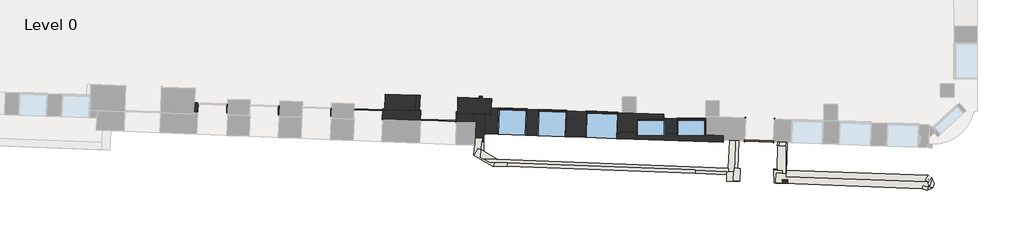
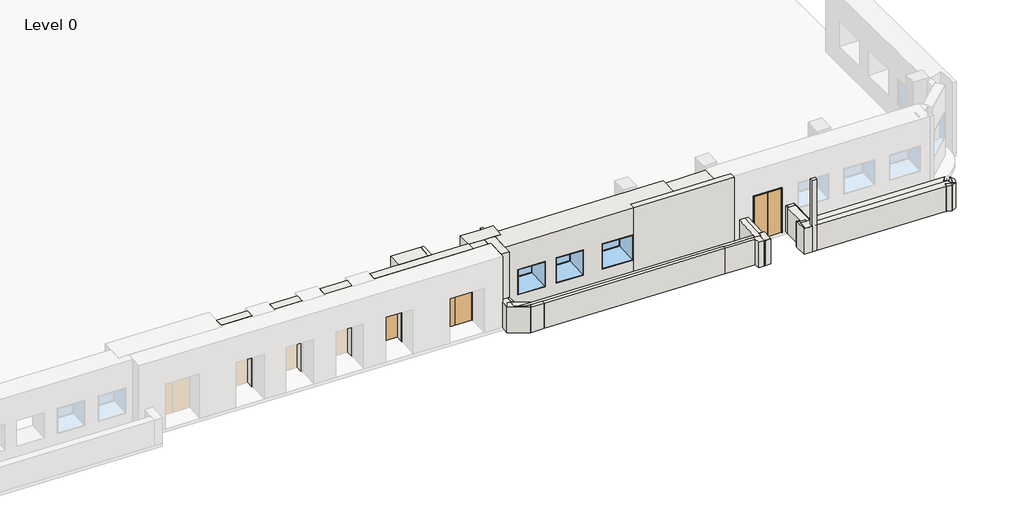
# One storey, part 2 of 9: 37 walls, 5 windows, 3 doors.
"""IFC4 building model written with IfcOpenShell, lengths in millimetres."""

import ifcopenshell
import ifcopenshell.guid

model = None  # the IFC model being written
_history = None  # IfcOwnerHistory: only IFC2X3 demands one
_inside = {}  # id of a spatial element -> (the spatial element, [elements in it])
_under = {}  # id of a project, library or spatial element -> (it, [spatial elements below it])
_declared = {}  # id of a project -> (the project, [libraries it declares])
_typed = {}  # id of a type object -> (the type object, [elements of that type])
_made_of = {}  # id of a material, layer set ... -> (it, [elements and type objects made of it])


def new_model(schema):
    """Start an empty IFC model of exactly this schema.

    Asked for "IFC4X3", IfcOpenShell would pick the latest addendum, in which some entities
    have other attributes; the version numbers below select the first issue.
    IFC2X3 requires an IfcOwnerHistory on every rooted entity: one is made here for all.
    """
    global model, _history
    if schema == "IFC4X3":
        model = ifcopenshell.file(schema_version=(4, 3, 0, 0))
    else:
        model = ifcopenshell.file(schema=schema)
    _inside.clear()
    _under.clear()
    _declared.clear()
    _typed.clear()
    _made_of.clear()
    _history = None
    if model.schema == "IFC2X3":
        org = make("IfcOrganization", Name="unknown")
        user = make(
            "IfcPersonAndOrganization",
            ThePerson=make("IfcPerson", FamilyName="unknown"),
            TheOrganization=org,
        )
        app = make(
            "IfcApplication",
            ApplicationDeveloper=org,
            Version="unknown",
            ApplicationFullName="unknown",
            ApplicationIdentifier="unknown",
        )
        _history = make(
            "IfcOwnerHistory",
            OwningUser=user,
            OwningApplication=app,
            ChangeAction="ADDED",
            CreationDate=0,
        )
    return model


def make(cls, **values):
    """One entity of the class cls with the attributes given. An attribute that is None is left unset."""
    return model.create_entity(
        cls, **{name: value for name, value in values.items() if value is not None}
    )


def rooted(cls, **values):
    """An entity with a GlobalId (a new one), such as an element, a storey or a relation."""
    return make(cls, GlobalId=ifcopenshell.guid.new(), OwnerHistory=_history, **values)


def si_unit(unit_type, name, prefix=None):
    """IfcSIUnit, for example si_unit("LENGTHUNIT", "METRE", prefix="MILLI")."""
    return make("IfcSIUnit", UnitType=unit_type, Prefix=prefix, Name=name)


def assignment(units):
    """IfcUnitAssignment: the units of a project."""
    return None if units is None else make("IfcUnitAssignment", Units=units)


def point(xyz):
    """IfcCartesianPoint."""
    return None if xyz is None else make("IfcCartesianPoint", Coordinates=xyz)


def direction(xyz):
    """IfcDirection."""
    return None if xyz is None else make("IfcDirection", DirectionRatios=xyz)


def frame(location, z_axis=None, x_axis=None):
    """IfcAxis2Placement3D, a coordinate frame: its origin and axes. An axis left out is left unset."""
    return make(
        "IfcAxis2Placement3D",
        Location=point(location),
        Axis=direction(z_axis),
        RefDirection=direction(x_axis),
    )


def origin():
    """The frame at (0, 0, 0) with its axes left unset."""
    return frame((0.0, 0.0, 0.0))


def origin_with_axes():
    """The frame at (0, 0, 0) with the z axis (0, 0, 1) and the x axis (1, 0, 0) written out."""
    return frame((0.0, 0.0, 0.0), z_axis=(0.0, 0.0, 1.0), x_axis=(1.0, 0.0, 0.0))


def place(relative_to, where):
    """IfcLocalPlacement: puts the frame where relative to a parent placement (None: the world)."""
    return make(
        "IfcLocalPlacement", PlacementRelTo=relative_to, RelativePlacement=where
    )


def context(
    kind, dimensions, precision=None, world=None, true_north=None, identifier=None
):
    """IfcGeometricRepresentationContext, for example the 3D "Model" context."""
    return make(
        "IfcGeometricRepresentationContext",
        ContextIdentifier=identifier,
        ContextType=kind,
        CoordinateSpaceDimension=dimensions,
        Precision=precision,
        WorldCoordinateSystem=world,
        TrueNorth=true_north,
    )


def project(units=None, contexts=None):
    """IfcProject with its units and contexts."""
    return rooted(
        "IfcProject",
        Name="project",
        RepresentationContexts=contexts,
        UnitsInContext=assignment(units),
    )


def spatial(cls, under=None, at=None, **own):
    """A site, building, storey or space (cls), placed at a placement, below another one or the project."""
    s = rooted(cls, ObjectPlacement=at, **own)
    if under is not None:
        _under.setdefault(under.id(), (under, []))[1].append(s)
    return s


def polyline(points):
    """IfcPolyline through the points."""
    return make("IfcPolyline", Points=[point(p) for p in points])


def outline(outer, holes=None, kind="AREA"):
    """IfcArbitraryClosedProfileDef: a profile drawn as a closed curve; with holes, ...WithVoids."""
    if holes is None:
        return make("IfcArbitraryClosedProfileDef", ProfileType=kind, OuterCurve=outer)
    return make(
        "IfcArbitraryProfileDefWithVoids",
        ProfileType=kind,
        OuterCurve=outer,
        InnerCurves=holes,
    )


def extrude(swept, where, along, depth):
    """IfcExtrudedAreaSolid: the profile swept, set in the frame where, extruded along a direction by depth."""
    return make(
        "IfcExtrudedAreaSolid",
        SweptArea=swept,
        Position=where,
        ExtrudedDirection=direction(along),
        Depth=depth,
    )


def faces_of(points, faces, orient=None, outer=None):
    """IfcFace entities. A face is a list of loops; a loop is a list of indices into points, from 0.

    orient and outer hold one flag for each loop. By default every Orientation is true, the
    first loop of a face is its IfcFaceOuterBound and the others are IfcFaceBound.
    """
    made = []
    for i, loops in enumerate(faces):
        bounds = []
        for j, loop in enumerate(loops):
            is_outer = j == 0 if outer is None else outer[i][j]
            bounds.append(
                make(
                    "IfcFaceOuterBound" if is_outer else "IfcFaceBound",
                    Bound=make("IfcPolyLoop", Polygon=[points[k] for k in loop]),
                    Orientation=True if orient is None else orient[i][j],
                )
            )
        made.append(make("IfcFace", Bounds=bounds))
    return made


def faceted_brep(points, faces, orient=None, outer=None, voids=None):
    """IfcFacetedBrep: a solid bounded by flat faces; with voids (closed shells), ...WithVoids."""
    shared = [point(p) for p in points]
    hull = make("IfcClosedShell", CfsFaces=faces_of(shared, faces, orient, outer))
    if voids is None:
        return make("IfcFacetedBrep", Outer=hull)
    return make(
        "IfcFacetedBrepWithVoids",
        Outer=hull,
        Voids=[
            make(cls, CfsFaces=faces_of(shared, fs, o, b)) for cls, fs, o, b in voids
        ],
    )


def shape(context_of_items, identifier, shape_type, items):
    """IfcShapeRepresentation: the items that make up one representation, for example the "Body"."""
    return make(
        "IfcShapeRepresentation",
        ContextOfItems=context_of_items,
        RepresentationIdentifier=identifier,
        RepresentationType=shape_type,
        Items=items,
    )


def source(mapping_origin, context_of_items, identifier, shape_type, items):
    """IfcRepresentationMap: a shape defined once, which mapped items show again and again."""
    return make(
        "IfcRepresentationMap",
        MappingOrigin=mapping_origin,
        MappedRepresentation=shape(context_of_items, identifier, shape_type, items),
    )


def transform(
    local_origin,
    x_axis=None,
    y_axis=None,
    z_axis=None,
    scale=None,
    scale2=None,
    scale3=None,
    uniform=True,
):
    """IfcCartesianTransformationOperator3D, or its non-uniform kind. x_axis, y_axis, z_axis: its Axis1, 2, 3."""
    if uniform:
        return make(
            "IfcCartesianTransformationOperator3D",
            Axis1=direction(x_axis),
            Axis2=direction(y_axis),
            LocalOrigin=point(local_origin),
            Scale=scale,
            Axis3=direction(z_axis),
        )
    return make(
        "IfcCartesianTransformationOperator3DnonUniform",
        Axis1=direction(x_axis),
        Axis2=direction(y_axis),
        LocalOrigin=point(local_origin),
        Scale=scale,
        Axis3=direction(z_axis),
        Scale2=scale2,
        Scale3=scale3,
    )


def mapped(mapping_source, mapping_target):
    """IfcMappedItem: shows the shape of a source again, moved by a transform."""
    return make(
        "IfcMappedItem", MappingSource=mapping_source, MappingTarget=mapping_target
    )


def made_of(thing, what):
    """Note that an element or type object is made of a material, layer set ...; save() writes the relation."""
    if what is not None:
        _made_of.setdefault(what.id(), (what, []))[1].append(thing)
    return thing


def element(
    cls,
    number,
    at=None,
    inside=None,
    cuts=None,
    type_object=None,
    material=None,
    context=None,
    identifier="Body",
    shape_type=None,
    held_by="IfcProductDefinitionShape",
    body=None,
    shapes=None,
    **own,
):
    """One element of the class cls, such as IfcWall. Its Tag is "e" and its number.

    at: its placement. inside: the storey or other place that contains it. cuts: it is an
    opening in that element (IfcRelVoidsElement). A single representation is given by context,
    identifier, shape_type and body (its items); several are given by shapes. held_by: the class
    of the entity that holds the representations. save() writes the other relations.
    """
    e = rooted(cls, Tag="e%d" % number, ObjectPlacement=at, **own)
    if body is not None:
        shapes = [shape(context, identifier, shape_type, body)]
    if shapes is not None:
        e.Representation = make(held_by, Representations=shapes)
    if inside is not None:
        _inside.setdefault(inside.id(), (inside, []))[1].append(e)
    if cuts is not None:
        rooted(
            "IfcRelVoidsElement", RelatingBuildingElement=cuts, RelatedOpeningElement=e
        )
    if type_object is not None:
        _typed.setdefault(type_object.id(), (type_object, []))[1].append(e)
    return made_of(e, material)


def aggregate(whole, parts):
    """IfcRelAggregates: a whole, such as a stair, and the parts it consists of."""
    return rooted("IfcRelAggregates", RelatingObject=whole, RelatedObjects=parts)


def save(model, path):
    """Write the relations noted so far, then the file.

    IfcRelAggregates (storeys below a building ...), IfcRelContainedInSpatialStructure (elements
    in a storey), IfcRelDefinesByType, IfcRelAssociatesMaterial and IfcRelDeclares: one each for
    every whole, place, type object, material and project.
    """
    for whole, parts in _under.values():
        aggregate(whole, parts)
    for where, things in _inside.values():
        rooted(
            "IfcRelContainedInSpatialStructure",
            RelatedElements=things,
            RelatingStructure=where,
        )
    for kind, things in _typed.values():
        rooted("IfcRelDefinesByType", RelatedObjects=things, RelatingType=kind)
    for what, things in _made_of.values():
        rooted("IfcRelAssociatesMaterial", RelatedObjects=things, RelatingMaterial=what)
    for by, libraries in _declared.values():
        rooted("IfcRelDeclares", RelatingContext=by, RelatedDefinitions=libraries)
    model.write(path)


def door_1200x2100mm_edb93628(model_context):
    return source(origin(), model_context, "Body", "SweptSolid", [
        extrude(outline(polyline([(2125.0, -625.0), (0.0, -625.0), (0.0, -600.0), (2100.0, -600.0), (2100.0, 600.0), (0.0, 600.0), (0.0, 625.0), (2125.0, 625.0), (2125.0, -625.0)])), frame((0.0, 195.0, 0.0), z_axis=(0.0, 1.0, 0.0), x_axis=(0.0, 0.0, 1.0)), (0.0, 0.0, 1.0), 30.0),
        extrude(outline(polyline([(2125.0, 625.0), (2125.0, -625.0), (0.0, -625.0), (0.0, -600.0), (2100.0, -600.0), (2100.0, 600.0), (0.0, 600.0), (0.0, 625.0), (2125.0, 625.0)])), frame((0.0, -225.0, 0.0), z_axis=(0.0, 1.0, 0.0), x_axis=(0.0, 0.0, 1.0)), (0.0, 0.0, 1.0), 30.0),
        extrude(outline(polyline([(600.0, 145.0), (-600.0, 145.0), (-600.0, 195.0), (600.0, 195.0), (600.0, 145.0)])), origin_with_axes(), (0.0, 0.0, 1.0), 2100.0),
    ])


def door_1200x2100mm_3dafc3e4(model_context):
    return source(origin(), model_context, "Body", "SweptSolid", [
        extrude(outline(polyline([(0.0, 485.0), (600.0, 485.0), (600.0, 435.0), (0.0, 435.0), (0.0, 485.0)])), origin_with_axes(), (0.0, 0.0, 1.0), 2100.0),
        extrude(outline(polyline([(-600.0, 485.0), (0.0, 485.0), (0.0, 435.0), (-600.0, 435.0), (-600.0, 485.0)])), origin_with_axes(), (0.0, 0.0, 1.0), 2100.0),
        extrude(outline(polyline([(2100.0, -600.0), (2100.0, 600.0), (0.0, 600.0), (0.0, 625.0), (2125.0, 625.0), (2125.0, -625.0), (0.0, -625.0), (0.0, -600.0), (2100.0, -600.0)])), frame((0.0, -510.0, 0.0), z_axis=(0.0, 1.0, 0.0), x_axis=(0.0, 0.0, 1.0)), (0.0, 0.0, 1.0), 25.0),
        extrude(outline(polyline([(2100.0, -600.0), (2100.0, 600.0), (0.0, 600.0), (0.0, 625.0), (2125.0, 625.0), (2125.0, -625.0), (0.0, -625.0), (0.0, -600.0), (2100.0, -600.0)])), frame((0.0, 485.0, 0.0), z_axis=(0.0, 1.0, 0.0), x_axis=(0.0, 0.0, 1.0)), (0.0, 0.0, 1.0), 25.0),
    ])


def door_1500x2100mm_1360b9d6(model_context):
    return source(origin(), model_context, "Body", "SweptSolid", [
        extrude(outline(polyline([(0.0, 195.0), (750.0, 195.0), (750.0, 145.0), (0.0, 145.0), (0.0, 195.0)])), origin_with_axes(), (0.0, 0.0, 1.0), 2100.0),
        extrude(outline(polyline([(-750.0, 195.0), (0.0, 195.0), (0.0, 145.0), (-750.0, 145.0), (-750.0, 195.0)])), origin_with_axes(), (0.0, 0.0, 1.0), 2100.0),
        extrude(outline(polyline([(2100.0, -750.0), (2100.0, 750.0), (0.0, 750.0), (0.0, 775.0), (2125.0, 775.0), (2125.0, -775.0), (0.0, -775.0), (0.0, -750.0), (2100.0, -750.0)])), frame((0.0, -220.0, 0.0), z_axis=(0.0, 1.0, 0.0), x_axis=(0.0, 0.0, 1.0)), (0.0, 0.0, 1.0), 25.0),
        extrude(outline(polyline([(2100.0, -750.0), (2100.0, 750.0), (0.0, 750.0), (0.0, 775.0), (2125.0, 775.0), (2125.0, -775.0), (0.0, -775.0), (0.0, -750.0), (2100.0, -750.0)])), frame((0.0, 195.0, 0.0), z_axis=(0.0, 1.0, 0.0), x_axis=(0.0, 0.0, 1.0)), (0.0, 0.0, 1.0), 25.0),
    ])


def window_instance_600x1200_86a208f5(model_context):
    return source(origin(), model_context, "Body", "SweptSolid", [
        extrude(outline(polyline([(-713.1, 567.9), (636.9, 567.9), (636.9, 542.5), (-713.1, 542.5), (-713.1, 567.9)])), frame((0.0, 0.0, 900.0), z_axis=(0.0, 0.0, 1.0), x_axis=(1.0, 0.0, 0.0)), (0.0, 0.0, 1.0), 19.05),
        extrude(outline(polyline([(573.4, 493.925), (-649.6, 493.925), (-649.6, 506.625), (573.4, 506.625), (573.4, 493.925)])), frame((0.0, 0.0, 963.5), z_axis=(0.0, 0.0, 1.0), x_axis=(1.0, 0.0, 0.0)), (0.0, 0.0, 1.0), 1073.0),
        extrude(outline(polyline([(2080.95, -694.05), (919.05, -694.05), (919.05, 617.85), (2080.95, 617.85), (2080.95, -694.05)]), holes=[polyline([(2036.5, -649.6), (2036.5, 573.4), (963.5, 573.4), (963.5, -649.6), (2036.5, -649.6)])]), frame((0.0, 478.05, 0.0), z_axis=(0.0, 1.0, 0.0), x_axis=(0.0, 0.0, 1.0)), (0.0, 0.0, 1.0), 44.45),
        extrude(outline(polyline([(2100.0, -713.1), (900.0, -713.1), (900.0, 636.9), (2100.0, 636.9), (2100.0, -713.1)]), holes=[polyline([(2068.25, -681.35), (2068.25, 605.15), (931.75, 605.15), (931.75, -681.35), (2068.25, -681.35)])]), frame((0.0, -542.5, 0.0), z_axis=(0.0, 1.0, 0.0), x_axis=(0.0, 0.0, 1.0)), (0.0, 0.0, 1.0), 1020.55),
        extrude(outline(polyline([(2100.0, 636.9), (2100.0, -713.1), (900.0, -713.1), (900.0, 636.9), (2100.0, 636.9)]), holes=[polyline([(2080.95, 617.85), (919.05, 617.85), (919.05, -694.05), (2080.95, -694.05), (2080.95, 617.85)])]), frame((0.0, 478.05, 0.0), z_axis=(0.0, 1.0, 0.0), x_axis=(0.0, 0.0, 1.0)), (0.0, 0.0, 1.0), 64.45),
    ])


def window_instance_600x1200_c70fa3c9(model_context):
    return source(origin(), model_context, "Body", "SweptSolid", [
        extrude(outline(polyline([(-638.1, 382.9), (561.9, 382.9), (561.9, 357.5), (-638.1, 357.5), (-638.1, 382.9)])), frame((0.0, 0.0, 900.0), z_axis=(0.0, 0.0, 1.0), x_axis=(1.0, 0.0, 0.0)), (0.0, 0.0, 1.0), 19.05),
        extrude(outline(polyline([(498.4, 308.925), (-574.6, 308.925), (-574.6, 321.625), (498.4, 321.625), (498.4, 308.925)])), frame((0.0, 0.0, 963.5), z_axis=(0.0, 0.0, 1.0), x_axis=(1.0, 0.0, 0.0)), (0.0, 0.0, 1.0), 1073.0),
        extrude(outline(polyline([(2080.95, -619.05), (919.05, -619.05), (919.05, 542.85), (2080.95, 542.85), (2080.95, -619.05)]), holes=[polyline([(2036.5, -574.6), (2036.5, 498.4), (963.5, 498.4), (963.5, -574.6), (2036.5, -574.6)])]), frame((0.0, 293.05, 0.0), z_axis=(0.0, 1.0, 0.0), x_axis=(0.0, 0.0, 1.0)), (0.0, 0.0, 1.0), 44.45),
        extrude(outline(polyline([(2100.0, -638.1), (900.0, -638.1), (900.0, 561.9), (2100.0, 561.9), (2100.0, -638.1)]), holes=[polyline([(2068.25, -606.35), (2068.25, 530.15), (931.75, 530.15), (931.75, -606.35), (2068.25, -606.35)])]), frame((0.0, -357.5, 0.0), z_axis=(0.0, 1.0, 0.0), x_axis=(0.0, 0.0, 1.0)), (0.0, 0.0, 1.0), 650.55),
        extrude(outline(polyline([(2100.0, 561.9), (2100.0, -638.1), (900.0, -638.1), (900.0, 561.9), (2100.0, 561.9)]), holes=[polyline([(2080.95, 542.85), (919.05, 542.85), (919.05, -619.05), (2080.95, -619.05), (2080.95, 542.85)])]), frame((0.0, 293.05, 0.0), z_axis=(0.0, 1.0, 0.0), x_axis=(0.0, 0.0, 1.0)), (0.0, 0.0, 1.0), 64.45),
    ])


def window_instance_600x1200_b5ab94bb(model_context):
    return source(origin(), model_context, "Body", "SweptSolid", [
        extrude(outline(polyline([(-638.1, 567.9), (561.9, 567.9), (561.9, 542.5), (-638.1, 542.5), (-638.1, 567.9)])), frame((0.0, 0.0, 900.0), z_axis=(0.0, 0.0, 1.0), x_axis=(1.0, 0.0, 0.0)), (0.0, 0.0, 1.0), 19.05),
        extrude(outline(polyline([(498.4, 493.925), (-574.6, 493.925), (-574.6, 506.625), (498.4, 506.625), (498.4, 493.925)])), frame((0.0, 0.0, 963.5), z_axis=(0.0, 0.0, 1.0), x_axis=(1.0, 0.0, 0.0)), (0.0, 0.0, 1.0), 1073.0),
        extrude(outline(polyline([(2080.95, -619.05), (919.05, -619.05), (919.05, 542.85), (2080.95, 542.85), (2080.95, -619.05)]), holes=[polyline([(2036.5, -574.6), (2036.5, 498.4), (963.5, 498.4), (963.5, -574.6), (2036.5, -574.6)])]), frame((0.0, 478.05, 0.0), z_axis=(0.0, 1.0, 0.0), x_axis=(0.0, 0.0, 1.0)), (0.0, 0.0, 1.0), 44.45),
        extrude(outline(polyline([(2100.0, -638.1), (900.0, -638.1), (900.0, 561.9), (2100.0, 561.9), (2100.0, -638.1)]), holes=[polyline([(2068.25, -606.35), (2068.25, 530.15), (931.75, 530.15), (931.75, -606.35), (2068.25, -606.35)])]), frame((0.0, -542.5, 0.0), z_axis=(0.0, 1.0, 0.0), x_axis=(0.0, 0.0, 1.0)), (0.0, 0.0, 1.0), 1020.55),
        extrude(outline(polyline([(2100.0, 561.9), (2100.0, -638.1), (900.0, -638.1), (900.0, 561.9), (2100.0, 561.9)]), holes=[polyline([(2080.95, 542.85), (919.05, 542.85), (919.05, -619.05), (2080.95, -619.05), (2080.95, 542.85)])]), frame((0.0, 478.05, 0.0), z_axis=(0.0, 1.0, 0.0), x_axis=(0.0, 0.0, 1.0)), (0.0, 0.0, 1.0), 64.45),
    ])


model = new_model("IFC4")

# Units and contexts
model_context = context("Model", 3, world=origin())
ifc_project = project(units=[si_unit("LENGTHUNIT", "METRE", prefix="MILLI")], contexts=[model_context])

# Site, building, storey
site = spatial("IfcSite", under=ifc_project)
building = spatial("IfcBuilding", under=site)
storey = spatial("IfcBuildingStorey", under=building, Name="Level 0", Elevation=0.0)

# Doors
placement = place(None, origin())
door_1200x2100mm_shape = door_1200x2100mm_edb93628(model_context)
element("IfcDoor", 1, ObjectType="1200x2100mm", at=placement, inside=storey, context=model_context, shape_type="MappedRepresentation", body=[
    mapped(door_1200x2100mm_shape, transform((29631.4891159, -6705.8487252, 0.0), x_axis=(0.9993300991115273, -0.03659717215503007, 0.0), y_axis=(0.03659717215503007, 0.9993300991115273, 0.0), z_axis=(0.0, 0.0, 1.0))),
])
door_1200x2100mm_2_shape = door_1200x2100mm_3dafc3e4(model_context)
element("IfcDoor", 2, ObjectType="1200x2100mm", at=placement, inside=storey, context=model_context, shape_type="MappedRepresentation", body=[
    mapped(door_1200x2100mm_2_shape, transform((46060.189886, -7389.4120026, 0.0), x_axis=(-0.9993300991327344, 0.03659717157594634, 0.0), y_axis=(-0.03659717157594634, -0.9993300991327344, 0.0), z_axis=(0.0, 0.0, 1.0))),
])
door_1500x2100mm_shape = door_1500x2100mm_1360b9d6(model_context)
element("IfcDoor", 3, ObjectType="1500x2100mm", at=placement, inside=storey, context=model_context, shape_type="MappedRepresentation", body=[
    mapped(door_1500x2100mm_shape, transform((32572.6767771, -6813.5600323, 0.0), x_axis=(-0.9993300991115273, 0.03659717215503007, 0.0), y_axis=(-0.03659717215503007, -0.9993300991115273, 0.0), z_axis=(0.0, 0.0, 1.0))),
])

# Walls
element("IfcWall", 4, at=placement, inside=storey, context=model_context, shape_type="Brep", body=[
    faceted_brep([(43803.0, -6920.4246385, 0.0), (42028.3722114, -6920.4246385, 0.0), (42028.3722114, -6920.4246385, 900.0), (42102.9199601, -6920.4246385, 900.0), (42102.9199601, -6920.4246385, 2100.0), (42028.3722114, -6920.4246385, 2100.0), (42028.3722114, -6920.4246385, 3350.0), (43803.0, -6920.4246385, 3350.0), (42588.0, -6920.4246385, 900.0), (43788.0, -6920.4246385, 900.0), (43788.0, -6920.4246385, 2100.0), (42588.0, -6920.4246385, 2100.0), (43803.0, -7596.9970274, 0.0), (42028.3722114, -7532.0071329, 0.0), (42028.3722114, -7532.0071329, 900.0), (42028.3722114, -7532.0071329, 2100.0), (42028.3722114, -7532.0071329, 3350.0), (43803.0, -7596.9970274, 3350.0), (42588.0, -7552.5016564, 900.0), (43788.0, -7596.4477018, 900.0), (42588.0, -7552.5016564, 2100.0), (43788.0, -7596.4477018, 2100.0), (42102.9199601, -7534.7371986, 900.0), (42102.9199601, -7534.7371986, 2100.0)], [[[0, 1, 2, 3, 4, 5, 6, 7], [8, 9, 10, 11]], [[1, 0, 12, 13]], [[2, 1, 13, 14]], [[6, 5, 15, 16]], [[7, 6, 16, 17]], [[0, 7, 17, 12]], [[9, 8, 18, 19]], [[8, 11, 20, 18]], [[11, 10, 21, 20]], [[10, 9, 19, 21]], [[4, 3, 22, 23]], [[3, 2, 14, 22]], [[5, 4, 23, 15]], [[13, 12, 17, 16, 15, 23, 22, 14], [19, 18, 20, 21]]]),
])
element("IfcWall", 5, at=placement, inside=storey, context=model_context, shape_type="Brep", body=[
    faceted_brep([(42048.226177, -6735.7880597, 3350.0), (42048.226177, -6735.7880597, 0.0), (40661.2576321, -6684.9949076, 0.0), (40306.4893089, -6672.0026869, 0.0), (34791.097467, -6470.0196367, 0.0), (34791.097467, -6470.0196367, 3350.0), (40306.4893089, -6672.0026869, 3350.0), (40661.2576321, -6684.9949076, 3350.0), (36298.9256684, -6525.2388755, 900.0), (36298.9256684, -6525.2388755, 2100.0), (35099.7295495, -6481.3222696, 2100.0), (35099.7295495, -6481.3222696, 900.0), (40134.0291636, -6665.6869024, 900.0), (40134.0291636, -6665.6869024, 2100.0), (38784.9335298, -6616.2807208, 2100.0), (38784.9335298, -6616.2807208, 900.0), (37970.7202035, -6586.4628409, 900.0), (37970.7202035, -6586.4628409, 2100.0), (36771.5240845, -6542.546235, 2100.0), (36771.5240845, -6542.546235, 900.0), (34483.8382747, -7544.494611, 3350.0), (34483.8382747, -7544.494611, 0.0), (40142.9656973, -7751.7415032, 0.0), (40142.9656973, -7751.7415032, 3350.0), (36259.2177373, -7609.5120331, 2100.0), (36259.2177373, -7609.5120331, 900.0), (35060.0216183, -7565.5954272, 900.0), (35060.0216183, -7565.5954272, 2100.0), (37931.0122723, -7670.7359985, 900.0), (36731.8161533, -7626.8193926, 900.0), (36731.8161533, -7626.8193926, 2100.0), (37931.0122723, -7670.7359985, 2100.0), (40094.3212324, -7749.9600599, 2100.0), (40094.3212324, -7749.9600599, 900.0), (38745.2255986, -7700.5538783, 900.0), (38745.2255986, -7700.5538783, 2100.0), (42019.07974, -7531.6668268, 0.0), (40153.5271914, -7463.3471126, 0.0), (34512.4814855, -6734.7416285, 0.0), (34778.2744561, -6747.0447242, 0.0), (34778.2744561, -6747.0447242, 3350.0), (34512.4814855, -6734.7416285, 3350.0), (40153.5271914, -7463.3471126, 3350.0), (42019.07974, -7531.6668268, 3350.0), (42019.07974, -7531.6668268, 2100.0), (42041.4644708, -6920.4246385, 2100.0), (42041.4644708, -6920.4246385, 900.0), (42019.07974, -7531.6668268, 900.0), (40902.9199601, -6920.4246385, 2100.0), (40902.9199601, -6920.4246385, 900.0), (40902.9199601, -7490.7911532, 900.0), (40902.9199601, -7490.7911532, 2100.0)], [[[0, 1, 2, 3, 4, 5, 6, 7], [8, 9, 10, 11], [12, 13, 14, 15], [16, 17, 18, 19]], [[20, 21, 22, 23], [24, 25, 26, 27], [28, 29, 30, 31], [32, 33, 34, 35]], [[4, 3, 2, 1, 36, 37, 22, 21, 38, 39]], [[0, 7, 6, 5, 40, 41, 20, 23, 42, 43]], [[1, 0, 43, 44, 45, 46, 47, 36]], [[21, 20, 41, 38]], [[40, 39, 38, 41]], [[39, 40, 5, 4]], [[25, 24, 9, 8]], [[26, 25, 8, 11]], [[27, 26, 11, 10]], [[24, 27, 10, 9]], [[32, 13, 12, 33]], [[33, 12, 15, 34]], [[34, 15, 14, 35]], [[13, 32, 35, 14]], [[31, 17, 16, 28]], [[28, 16, 19, 29]], [[29, 19, 18, 30]], [[17, 31, 30, 18]], [[48, 49, 46, 45]], [[46, 49, 50, 47]], [[49, 48, 51, 50]], [[48, 45, 44, 51]], [[42, 37, 36, 47, 50, 51, 44, 43]], [[37, 42, 23, 22]]]),
])
element("IfcWall", 6, at=placement, inside=storey, context=model_context, shape_type="Brep", body=[
    faceted_brep([(34808.7920354, -6087.7506491, 0.0), (34420.0000015, -6069.7541402, 0.0), (34295.0000015, -6063.968107, 0.0), (33379.3663645, -6021.5850139, 0.0), (33379.3663645, -6021.5850139, 3350.0), (34295.0000015, -6063.968107, 3350.0), (34420.0000015, -6069.7541402, 3350.0), (34808.7920354, -6087.7506491, 3350.0), (34778.2744561, -6747.0447242, 0.0), (34778.2744561, -6747.0447242, 3350.0), (34512.4814855, -6734.7416285, 3350.0), (34039.3663645, -6712.8419501, 3350.0), (33379.3663645, -6682.2916947, 3350.0), (33379.3663645, -6682.2916947, 0.0), (34039.3663645, -6712.8419501, 0.0), (34512.4814855, -6734.7416285, 0.0), (34791.097467, -6470.0196367, 0.0), (33379.3663645, -6647.9716622, 0.0), (33379.3663645, -6647.9716622, 3350.0), (34791.097467, -6470.0196367, 3350.0)], [[[0, 1, 2, 3, 4, 5, 6, 7]], [[8, 9, 10, 11, 12, 13, 14, 15]], [[3, 2, 1, 0, 16, 8, 15, 14, 13, 17]], [[7, 6, 5, 4, 18, 12, 11, 10, 9, 19]], [[0, 7, 19, 9, 8, 16]], [[4, 3, 17, 13, 12, 18]]]),
])
element("IfcWall", 7, at=placement, inside=storey, context=model_context, shape_type="SweptSolid", body=[
    extrude(outline(polyline([(34039.3663645, -6712.8419501), (34039.3663645, -7036.0955505), (33870.2310482, -7036.0955505), (33379.3663645, -7016.639414), (33379.3663645, -6682.2916947), (34039.3663645, -6712.8419501)])), origin_with_axes(), (0.0, 0.0, 1.0), 3350.0),
])
element("IfcWall", 8, at=placement, inside=storey, context=model_context, shape_type="SweptSolid", body=[
    extrude(outline(polyline([(31803.7889856, -5937.0320064), (31778.914896, -6589.3604006), (31629.0152108, -6583.8708185), (31653.8857363, -5931.6358942), (31803.7889856, -5937.0320064)])), origin_with_axes(), (0.0, 0.0, 1.0), 3350.0),
])
element("IfcWall", 9, at=placement, inside=storey, context=model_context, shape_type="SweptSolid", body=[
    extrude(outline(polyline([(30346.5613741, -5884.5757468), (31653.8857363, -5931.6358942), (31629.0152108, -6583.8708185), (30323.1101913, -6536.04635), (30346.5613741, -5884.5757468)])), origin_with_axes(), (0.0, 0.0, 1.0), 3350.0),
])
element("IfcWall", 10, at=placement, inside=storey, context=model_context, shape_type="Brep", body=[
    faceted_brep([(46725.7179376, -9608.4296632, 1200.0), (46725.7179376, -9608.4296632, 0.0), (47034.9573377, -9621.391772, 0.0), (52882.4973637, -9866.4978283, 0.0), (52882.4973637, -9866.4978283, 1200.0), (47034.9573377, -9621.391772, 1200.0), (46743.3072533, -9188.7981392, 0.0), (46743.3072533, -9188.7981392, 1200.0), (46813.0780657, -9191.7226594, 1200.0), (47013.7377301, -9200.1335294, 1200.0), (47132.8075582, -9205.1244719, 1200.0), (47162.9417406, -9206.3875792, 1200.0), (47162.9417406, -9206.3875792, 0.0), (47132.8075582, -9205.1244719, 0.0), (47013.7377301, -9200.1335294, 0.0), (46813.0780657, -9191.7226594, 0.0), (47161.2704993, -9363.3223401, 0.0), (53106.1337632, -9570.3540362, 0.0), (53170.4080717, -9733.588106, 0.0), (53094.5456575, -9767.4192175, 0.0), (52912.9626558, -9719.3978943, 0.0), (52874.6121821, -9864.4125183, 0.0), (52874.6121821, -9864.4125183, 1200.0), (52912.9626558, -9719.3978943, 1200.0), (53094.5456575, -9767.4192175, 1200.0), (53170.4080717, -9733.588106, 1200.0), (53106.1337632, -9570.3540362, 1200.0), (47161.2704993, -9363.3223401, 1200.0)], [[[0, 1, 2, 3, 4, 5]], [[6, 7, 8, 9, 10, 11, 12, 13, 14, 15]], [[1, 6, 15, 14, 13, 12, 16, 17, 18, 19, 20, 21, 3, 2]], [[7, 0, 5, 4, 22, 23, 24, 25, 26, 27, 11, 10, 9, 8]], [[1, 0, 7, 6]], [[16, 27, 26, 17]], [[27, 16, 12, 11]], [[17, 26, 25, 18]], [[18, 25, 24, 19]], [[23, 20, 19, 24]], [[21, 22, 4, 3]], [[20, 23, 22, 21]]]),
    faceted_brep([(53145.1949713, -9457.1402873, 0.0), (53145.1949713, -9457.1402873, 1200.0), (53148.8000151, -9457.2913966, 1200.0), (53148.8000151, -9457.2913966, 0.0), (53145.1395137, -9458.7327391, 0.0), (53145.1395137, -9458.7327391, 1200.0)], [[[0, 1, 2, 3]], [[0, 3, 4]], [[2, 1, 5]], [[1, 0, 4, 5]], [[3, 2, 5, 4]]]),
])
element("IfcWall", 11, at=placement, inside=storey, context=model_context, shape_type="Brep", body=[
    faceted_brep([(46656.7562332, -9070.3441923, 0.0), (46684.1320088, -9613.8165976, 0.0), (46684.1320088, -9613.8165976, 1200.0), (46656.7562332, -9070.3441923, 1200.0), (47035.0903174, -9624.0317277, 1200.0), (47035.0903174, -9624.0317277, 0.0), (47034.9573377, -9621.391772, 0.0), (47034.9573377, -9621.391772, 1200.0), (47009.1282597, -9108.6248898, 0.0), (47009.1282597, -9108.6248898, 1200.0), (47013.7377301, -9200.1335294, 1200.0), (47013.7377301, -9200.1335294, 0.0), (46814.1885238, -9087.4471898, 0.0), (46743.3072533, -9188.7981392, 0.0), (46725.7179376, -9608.4296632, 0.0), (46725.7179376, -9608.4296632, 1200.0), (46743.3072533, -9188.7981392, 1200.0), (46814.1885238, -9087.4471898, 1200.0)], [[[0, 1, 2, 3]], [[4, 5, 6, 7]], [[8, 9, 10, 11]], [[1, 0, 12, 8, 11, 13, 14, 6, 5]], [[3, 2, 4, 7, 15, 16, 10, 9, 17]], [[2, 1, 5, 4]], [[0, 3, 17, 9, 8, 12]], [[14, 15, 7, 6]], [[16, 13, 11, 10]], [[15, 14, 13, 16]]]),
])
element("IfcWall", 12, at=placement, inside=storey, context=model_context, shape_type="Brep", body=[
    faceted_brep([(47035.0903174, -9624.0317277, 0.0), (47241.2250098, -9630.0315648, 0.0), (47241.2250098, -9630.0315648, 3350.0), (47035.0903174, -9624.0317277, 3350.0), (47035.0903174, -9624.0317277, 1200.0), (47027.5202232, -9473.7478644, 0.0), (47027.5202232, -9473.7478644, 3350.0), (47245.5891204, -9480.0950631, 3350.0), (47245.5891204, -9480.0950631, 0.0), (47034.9573377, -9621.391772, 0.0)], [[[0, 1, 2, 3, 4]], [[5, 6, 7, 8]], [[1, 0, 9, 5, 8]], [[2, 1, 8, 7]], [[3, 2, 7, 6]], [[0, 4, 3, 6, 5, 9]]]),
])
element("IfcWall", 13, at=placement, inside=storey, context=model_context, shape_type="Brep", body=[
    faceted_brep([(45050.3783928, -7837.7561042, 1200.0), (45050.3783928, -7837.7561042, 0.0), (45014.0988418, -8751.7129035, 0.0), (45004.3038415, -8998.4691866, 0.0), (45004.3038415, -8998.4691866, 1200.0), (45014.0988418, -8751.7129035, 1200.0), (45200.2786135, -7843.2457058, 0.0), (45200.2786135, -7843.2457058, 1200.0), (45154.1721064, -9004.7638203, 1200.0), (45154.1721064, -9004.7638203, 0.0)], [[[0, 1, 2, 3, 4, 5]], [[6, 7, 8, 9]], [[1, 6, 9, 3, 2]], [[7, 0, 5, 4, 8]], [[1, 0, 7, 6]], [[4, 3, 9, 8]]]),
])
element("IfcWall", 14, at=placement, inside=storey, context=model_context, shape_type="SweptSolid", body=[
    extrude(outline(polyline([(45226.5719008, -9534.7815961), (44986.5363305, -9534.297451), (44986.2023328, -9524.685807), (45226.5719008, -9534.7815961)])), origin_with_axes(), (0.0, 0.0, 1.0), 1200.0),
])
element("IfcWall", 15, at=placement, inside=storey, context=model_context, shape_type="Brep", body=[
    faceted_brep([(44696.3409547, -9533.7121351, 0.0), (44696.3409547, -9533.7121351, 1200.0), (44686.4521431, -9249.1361645, 1200.0), (44686.4521431, -9249.1361645, 0.0), (44986.5363305, -9534.297451, 1200.0), (44986.5363305, -9534.297451, 0.0), (44986.2023328, -9524.685807, 0.0), (44986.2023328, -9524.685807, 1200.0), (44691.2804268, -9137.2933698, 0.0), (44745.1826783, -9139.3772197, 0.0), (44952.5868699, -9147.395423, 0.0), (44936.8273564, -9522.6120031, 0.0), (44936.8273564, -9522.6120031, 1200.0), (44952.5868699, -9147.395423, 1200.0), (44745.1826783, -9139.3772197, 1200.0), (44691.2804268, -9137.2933698, 1200.0)], [[[0, 1, 2, 3]], [[4, 5, 6, 7]], [[5, 0, 3, 8, 9, 10, 11, 6]], [[1, 4, 7, 12, 13, 14, 15, 2]], [[1, 0, 5, 4]], [[8, 15, 14, 13, 10, 9]], [[3, 2, 15, 8]], [[12, 11, 10, 13]], [[11, 12, 7, 6]]]),
])
element("IfcWall", 16, at=placement, inside=storey, context=model_context, shape_type="Brep", body=[
    faceted_brep([(44808.1533154, -7828.885409, 0.0), (44752.3823604, -8989.5435063, 0.0), (44745.1826783, -9139.3772197, 0.0), (44745.1826783, -9139.3772197, 1200.0), (44752.3823604, -8989.5435063, 1200.0), (44808.1533154, -7828.885409, 1200.0), (44995.0070404, -9149.035378, 1200.0), (44995.0070404, -9149.035378, 0.0), (45002.2460719, -8998.3827579, 0.0), (45014.0988418, -8751.7129035, 0.0), (45014.0988418, -8751.7129035, 1200.0), (45002.2460719, -8998.3827579, 1200.0), (45050.3783928, -7837.7561042, 0.0), (44973.1193449, -9148.1892042, 0.0), (44952.5868699, -9147.395423, 0.0), (44952.5868699, -9147.395423, 1200.0), (44973.1193449, -9148.1892042, 1200.0), (45050.3783928, -7837.7561042, 1200.0)], [[[0, 1, 2, 3, 4, 5]], [[6, 7, 8, 9, 10, 11]], [[2, 1, 0, 12, 9, 8, 7, 13, 14]], [[5, 4, 3, 15, 16, 6, 11, 10, 17]], [[3, 2, 14, 13, 7, 6, 16, 15]], [[0, 5, 17, 12]], [[10, 9, 12, 17]]]),
])
element("IfcWall", 17, at=placement, inside=storey, context=model_context, shape_type="Brep", body=[
    faceted_brep([(44752.3823604, -8989.5435063, 0.0), (35052.3823604, -8614.5435063, 0.0), (34447.051082, -8591.1415239, 0.0), (34447.051082, -8591.1415239, 1200.0), (35052.3823604, -8614.5435063, 1200.0), (44752.3823604, -8989.5435063, 1200.0), (44745.1826783, -9139.3772197, 0.0), (44745.1826783, -9139.3772197, 1200.0), (44691.2804268, -9137.2933698, 1200.0), (43370.9400308, -9086.2492823, 1200.0), (43370.2927154, -9086.2242572, 1200.0), (43370.2927154, -9086.2242572, 0.0), (43370.9400308, -9086.2492823, 0.0), (44691.2804268, -9137.2933698, 0.0), (35457.2442549, -8780.3074353, 1200.0), (35457.2442549, -8780.3074353, 0.0), (35459.0397322, -8780.3768481, 0.0), (35459.0397322, -8780.3768481, 1200.0), (34716.1503877, -8751.6568992, 1200.0), (34716.1503877, -8751.6568992, 0.0), (34934.8078129, -8760.1101501, 0.0), (34934.8078129, -8760.1101501, 1200.0), (43371.0888614, -9064.7352056, 0.0), (35459.364371, -8771.6144098, 0.0), (35457.4359082, -8771.5575692, 0.0), (34942.975587, -8760.2890535, 0.0), (34942.975587, -8760.2890535, 1200.0), (35457.4359082, -8771.5575692, 1200.0), (35459.364371, -8771.6144098, 1200.0), (43371.0888614, -9064.7352056, 1200.0)], [[[0, 1, 2, 3, 4, 5]], [[6, 7, 8, 9, 10, 11, 12, 13]], [[14, 15, 16, 17]], [[18, 19, 20, 21]], [[2, 1, 0, 6, 13, 12, 11, 22, 23, 16, 15, 24, 25, 20, 19]], [[5, 4, 3, 18, 21, 26, 27, 14, 17, 28, 29, 10, 9, 8, 7]], [[0, 5, 7, 6]], [[3, 2, 19, 18]], [[24, 27, 26, 21, 20, 25]], [[27, 24, 15, 14]], [[28, 23, 22, 29]], [[23, 28, 17, 16]], [[29, 22, 11, 10]]]),
])
element("IfcWall", 18, at=placement, inside=storey, context=model_context, shape_type="Brep", body=[
    faceted_brep([(35052.3823604, -8614.5435063, 0.0), (34482.3823604, -8274.5435063, 0.0), (34372.4646051, -8208.9785294, 0.0), (34372.4646051, -8208.9785294, 1200.0), (34482.3823604, -8274.5435063, 1200.0), (35052.3823604, -8614.5435063, 1200.0), (34447.051082, -8591.1415239, 0.0), (34447.051082, -8591.1415239, 1200.0), (34342.2256033, -8528.6140454, 1200.0), (34342.2256033, -8528.6140454, 0.0), (34346.9699217, -8478.4651458, 0.0), (34370.7920008, -8226.65847, 0.0), (34370.7920008, -8226.65847, 1200.0), (34346.9699217, -8478.4651458, 1200.0)], [[[0, 1, 2, 3, 4, 5]], [[6, 7, 8, 9]], [[2, 1, 0, 6, 9, 10, 11]], [[5, 4, 3, 12, 13, 8, 7]], [[0, 5, 7, 6]], [[3, 2, 11, 10, 9, 8, 13, 12]]]),
])
element("IfcWall", 19, at=placement, inside=storey, context=model_context, shape_type="SweptSolid", body=[
    extrude(outline(polyline([(34481.6585107, -7912.1599464), (34482.3823604, -8274.5435063), (34372.4646051, -8208.9785294), (34400.5296883, -7912.3219987), (34481.6585107, -7912.1599464)])), origin_with_axes(), (0.0, 0.0, 1.0), 1200.0),
])
element("IfcWall", 20, at=placement, inside=storey, context=model_context, shape_type="Brep", body=[
    faceted_brep([(34470.6814303, -7916.4429278, 3350.0), (34470.6814303, -7916.4429278, 0.0), (34483.8382747, -7544.494611, 0.0), (34512.4814855, -6734.7416285, 0.0), (34512.4814855, -6734.7416285, 3350.0), (34483.8382747, -7544.494611, 3350.0), (34150.5080181, -7047.2047364, 0.0), (33870.2310482, -7036.0955505, 0.0), (34039.3663645, -7036.0955505, 0.0), (34039.3663645, -6712.8419501, 0.0), (34400.3751044, -7913.9559979, 0.0), (34416.6661555, -7741.7545955, 0.0), (34127.9552642, -7714.4412066, 0.0), (34121.253146, -7785.2846496, 0.0), (33870.2310482, -7036.0955505, 3350.0), (34150.5080181, -7047.2047364, 3350.0), (34116.5510057, -7903.9163517, 3350.0), (34039.3663645, -6712.8419501, 3350.0), (34039.3663645, -7036.0955505, 3350.0), (34116.5510057, -7903.9163517, 1200.0), (34400.3751044, -7913.9559979, 1200.0), (34416.6661555, -7741.7545955, 1200.0), (34127.9552642, -7714.4412066, 1200.0), (34121.253146, -7785.2846496, 1200.0)], [[[0, 1, 2, 3, 4, 5]], [[6, 7, 8, 9, 3, 2, 1, 10, 11, 12, 13]], [[14, 15, 16, 0, 5, 4, 17, 18]], [[1, 0, 16, 19, 20, 10]], [[6, 15, 14, 7]], [[8, 18, 17, 9]], [[18, 8, 7, 14]], [[4, 3, 9, 17]], [[21, 11, 10, 20]], [[12, 22, 23, 13]], [[11, 21, 22, 12]], [[22, 21, 20, 19, 23]], [[15, 6, 13, 23, 19, 16]]]),
])
element("IfcWall", 21, at=placement, inside=storey, context=model_context, shape_type="SweptSolid", body=[
    extrude(outline(polyline([(34295.0000015, -5968.9949076), (34420.0000015, -5968.9949076), (34420.0000015, -6069.7541402), (34295.0000015, -6063.968107), (34295.0000015, -5968.9949076)])), origin_with_axes(), (0.0, 0.0, 1.0), 3350.0),
])
element("IfcWall", 22, at=placement, inside=storey, context=model_context, shape_type="Brep", body=[
    faceted_brep([(44550.5796276, -7624.3746676, 0.0), (43803.0, -7596.9970274, 0.0), (43786.1100554, -7596.3784888, 0.0), (42028.3722114, -7532.0071329, 0.0), (42019.07974, -7531.6668268, 0.0), (40153.5271914, -7463.3471126, 0.0), (40153.5271914, -7463.3471126, 3350.0), (42019.07974, -7531.6668268, 3350.0), (42028.3722114, -7532.0071329, 3350.0), (43786.1100554, -7596.3784888, 3350.0), (43803.0, -7596.9970274, 3350.0), (44550.5796276, -7624.3746676, 3350.0), (42102.9199601, -7534.7371986, 900.0), (42102.9199601, -7534.7371986, 2100.0), (42028.3722114, -7532.0071329, 2100.0), (42019.07974, -7531.6668268, 2100.0), (40902.9199601, -7490.7911532, 2100.0), (40902.9199601, -7490.7911532, 900.0), (42019.07974, -7531.6668268, 900.0), (42028.3722114, -7532.0071329, 900.0), (43788.0, -7596.4477018, 900.0), (43788.0, -7596.4477018, 2100.0), (42588.0, -7552.5016564, 2100.0), (42588.0, -7552.5016564, 900.0), (40142.9140117, -7753.1528414, 0.0), (44539.9664478, -7914.1803963, 0.0), (44539.9664478, -7914.1803963, 3350.0), (40142.9140117, -7753.1528414, 3350.0), (44543.4451089, -7819.1913433, 0.0), (40142.9656973, -7751.7415032, 0.0), (40142.9656973, -7751.7415032, 3350.0), (44543.4451089, -7819.1913433, 3350.0), (40902.9199601, -7635.4246385, 2100.0), (42102.9199601, -7635.4246385, 2100.0), (42102.9199601, -7635.4246385, 900.0), (40902.9199601, -7635.4246385, 900.0), (42588.0, -7635.4246385, 2100.0), (43788.0, -7635.4246385, 2100.0), (43788.0, -7635.4246385, 900.0), (42588.0, -7635.4246385, 900.0)], [[[0, 1, 2, 3, 4, 5, 6, 7, 8, 9, 10, 11], [12, 13, 14, 15, 16, 17, 18, 19], [20, 21, 22, 23]], [[24, 25, 26, 27]], [[5, 4, 3, 2, 1, 0, 28, 25, 24, 29]], [[6, 5, 29, 24, 27, 30]], [[11, 10, 9, 8, 7, 6, 30, 27, 26, 31]], [[0, 11, 31, 26, 25, 28]], [[32, 33, 34, 35]], [[34, 33, 13, 12]], [[35, 34, 12, 19, 18, 17]], [[32, 35, 17, 16]], [[33, 32, 16, 15, 14, 13]], [[36, 37, 38, 39]], [[38, 37, 21, 20]], [[39, 38, 20, 23]], [[36, 39, 23, 22]], [[37, 36, 22, 21]]]),
])
element("IfcWall", 23, at=placement, inside=storey, context=model_context, shape_type="SweptSolid", body=[
    extrude(outline(polyline([(45093.7654502, -9022.7892164), (45069.6449584, -9010.7790807), (45089.7025928, -8970.496438), (45113.8230846, -8982.5065737), (45093.7654502, -9022.7892164)])), origin_with_axes(), (0.0, 0.0, 1.0), 1200.0),
])
element("IfcWall", 24, at=placement, inside=storey, context=model_context, shape_type="Brep", body=[
    faceted_brep([(44936.8273564, -9522.6120031, 0.0), (44936.8273564, -9522.6120031, 1200.0), (44952.5868699, -9147.395423, 1200.0), (44952.5868699, -9147.395423, 0.0), (45226.5719008, -9534.7815961, 0.0), (45248.6665396, -9008.7326915, 0.0), (45248.6665396, -9008.7326915, 1200.0), (45226.5719008, -9534.7815961, 1200.0), (44986.2023328, -9524.685807, 0.0), (44995.0070404, -9149.035378, 0.0), (45002.2460719, -8998.3827579, 0.0), (45004.3038415, -8998.4691866, 0.0), (45154.1721064, -9004.7638203, 0.0), (44986.2023328, -9524.685807, 1200.0), (45154.1721064, -9004.7638203, 1200.0), (45004.3038415, -8998.4691866, 1200.0), (45002.2460719, -8998.3827579, 1200.0), (44995.0070404, -9149.035378, 1200.0)], [[[0, 1, 2, 3]], [[4, 5, 6, 7]], [[5, 4, 8, 0, 3, 9, 10, 11, 12]], [[1, 0, 8, 4, 7, 13]], [[7, 6, 14, 15, 16, 17, 2, 1, 13]], [[6, 5, 12, 11, 10, 16, 15, 14]], [[9, 17, 16, 10]], [[17, 9, 3, 2]]]),
])
element("IfcWall", 25, at=placement, inside=storey, context=model_context, shape_type="Brep", body=[
    faceted_brep([(34416.6661555, -7741.7545955, 0.0), (34416.6661555, -7741.7545955, 1200.0), (34400.5296883, -7912.3219987, 1200.0), (34400.3751044, -7913.9559979, 1200.0), (34372.4646051, -8208.9785294, 1200.0), (34370.7920008, -8226.65847, 1200.0), (34370.7920008, -8226.65847, 0.0), (34372.4646051, -8208.9785294, 0.0), (34400.3751044, -7913.9559979, 0.0), (34400.5296883, -7912.3219987, 0.0), (34127.9552642, -7714.4412066, 0.0), (34121.253146, -7785.2846496, 0.0), (34058.2590304, -8451.1517569, 0.0), (34058.2590304, -8451.1517569, 1200.0), (34121.253146, -7785.2846496, 1200.0), (34127.9552642, -7714.4412066, 1200.0), (34231.9560418, -8147.2943097, 0.0), (34231.9560418, -8147.2943097, 1200.0)], [[[0, 1, 2, 3, 4, 5, 6, 7, 8, 9]], [[10, 11, 12, 13, 14, 15]], [[12, 11, 10, 0, 9, 8, 7, 6, 16]], [[1, 0, 10, 15]], [[15, 14, 13, 17, 5, 4, 3, 2, 1]], [[17, 16, 6, 5]], [[16, 17, 13, 12]]]),
])
element("IfcWall", 26, at=placement, inside=storey, context=model_context, shape_type="SweptSolid", body=[
    extrude(outline(polyline([(46883.1422894, -7905.4792038), (46877.6996835, -8054.0961498), (46817.7398775, -8051.9003196), (46823.1824835, -7903.2833735), (46883.1422894, -7905.4792038)])), origin_with_axes(), (0.0, 0.0, 1.0), 1200.0),
])
element("IfcWall", 27, at=placement, inside=storey, context=model_context, shape_type="Brep", body=[
    faceted_brep([(46877.6996835, -8054.0961498, 0.0), (47172.5164763, -8064.8928433, 0.0), (47172.5164763, -8064.8928433, 1200.0), (46877.6996835, -8054.0961498, 1200.0), (46883.1892593, -7904.196635, 0.0), (46883.1892593, -7904.196635, 1200.0), (47177.7371161, -7914.9834795, 1200.0), (47177.7371161, -7914.9834795, 0.0), (46883.1422894, -7905.4792038, 0.0), (47177.7134606, -7915.6627404, 0.0), (47177.7134606, -7915.6627404, 1200.0), (46883.1422894, -7905.4792038, 1200.0)], [[[0, 1, 2, 3]], [[4, 5, 6, 7]], [[1, 0, 8, 4, 7, 9]], [[3, 2, 10, 6, 5, 11]], [[0, 3, 11, 5, 4, 8]], [[2, 1, 9, 7, 6, 10]]]),
])
element("IfcWall", 28, at=placement, inside=storey, context=model_context, shape_type="Brep", body=[
    faceted_brep([(53145.6815546, -9780.9425837, 0.0), (53094.5456575, -9767.4192175, 0.0), (52912.9626558, -9719.3978943, 0.0), (52912.9626558, -9719.3978943, 1200.0), (53094.5456575, -9767.4192175, 1200.0), (53145.6815546, -9780.9425837, 1200.0), (53107.3310809, -9925.9572077, 0.0), (53107.3310809, -9925.9572077, 1200.0), (52882.4973637, -9866.4978283, 1200.0), (52874.6121821, -9864.4125183, 1200.0), (52874.6121821, -9864.4125183, 0.0), (52882.4973637, -9866.4978283, 0.0)], [[[0, 1, 2, 3, 4, 5]], [[6, 7, 8, 9, 10, 11]], [[2, 1, 0, 6, 11, 10]], [[3, 2, 10, 9]], [[5, 4, 3, 9, 8, 7]], [[0, 5, 7, 6]]]),
])
element("IfcWall", 29, at=placement, inside=storey, context=model_context, shape_type="SweptSolid", body=[
    extrude(outline(polyline([(53334.5728815, -9824.6179246), (53107.3310809, -9925.9572077), (53145.6815546, -9780.9425837), (53094.5456575, -9767.4192175), (53170.4080717, -9733.588106), (53207.3762133, -9827.4741444), (53220.524301, -9787.2960636), (53334.5728815, -9824.6179246)])), origin_with_axes(), (0.0, 0.0, 1.0), 1200.0),
])
element("IfcWall", 30, at=placement, inside=storey, context=model_context, shape_type="SweptSolid", body=[
    extrude(outline(polyline([(53220.524301, -9787.2960636), (53329.3248181, -9454.8221679), (53398.2794567, -9629.942625), (53334.5728815, -9824.6179246), (53220.524301, -9787.2960636)])), origin_with_axes(), (0.0, 0.0, 1.0), 1200.0),
])
element("IfcWall", 31, at=placement, inside=storey, context=model_context, shape_type="Brep", body=[
    faceted_brep([(53207.3762133, -9827.4741444, 0.0), (53207.3762133, -9827.4741444, 1200.0), (53170.4080717, -9733.588106, 1200.0), (53106.1337632, -9570.3540362, 1200.0), (53099.9900171, -9554.7510885, 1200.0), (53099.9900171, -9554.7510885, 0.0), (53106.1337632, -9570.3540362, 0.0), (53170.4080717, -9733.588106, 0.0), (53329.3248181, -9454.8221679, 0.0), (53305.9344392, -9395.418857, 0.0), (53305.9344392, -9395.418857, 1200.0), (53329.3248181, -9454.8221679, 1200.0), (53220.524301, -9787.2960636, 0.0), (53158.8593245, -9597.579463, 0.0), (53158.8593245, -9597.579463, 1200.0), (53220.524301, -9787.2960636, 1200.0)], [[[0, 1, 2, 3, 4, 5, 6, 7]], [[8, 9, 10, 11]], [[9, 8, 12, 0, 7, 6, 5, 13]], [[11, 10, 14, 4, 3, 2, 1, 15]], [[1, 0, 12, 8, 11, 15]], [[14, 13, 5, 4]], [[13, 14, 10, 9]]]),
])
element("IfcWall", 32, at=placement, inside=storey, context=model_context, shape_type="Brep", body=[
    faceted_brep([(47161.2704993, -9363.3223401, 1200.0), (47161.2704993, -9363.3223401, 0.0), (53106.1337632, -9570.3540362, 0.0), (53122.2062612, -9570.9137659, 0.0), (53122.2062612, -9570.9137659, 1200.0), (53106.1337632, -9570.3540362, 1200.0), (53151.3029481, -9281.751264, 1200.0), (53151.3029481, -9281.751264, 0.0), (53149.6129026, -9281.6924076, 0.0), (47164.3595154, -9073.254113, 0.0), (47164.3595154, -9073.254113, 1200.0), (53149.6129026, -9281.6924076, 1200.0), (47162.9417406, -9206.3875792, 0.0), (53002.5380558, -9483.8532086, 0.0), (53151.2631863, -9282.8930157, 0.0), (53151.2631863, -9282.8930157, 1200.0), (47162.9417406, -9206.3875792, 1200.0), (53002.5380558, -9483.8532086, 1200.0)], [[[0, 1, 2, 3, 4, 5]], [[6, 7, 8, 9, 10, 11]], [[1, 12, 9, 8, 13, 3, 2]], [[8, 7, 14]], [[7, 6, 15, 14]], [[10, 16, 0, 5, 4, 17, 11]], [[6, 11, 15]], [[1, 0, 16, 10, 9, 12]], [[13, 17, 4, 3]], [[11, 8, 14, 15]], [[17, 13, 8, 11]]]),
])
element("IfcWall", 33, at=placement, inside=storey, context=model_context, shape_type="Brep", body=[
    faceted_brep([(47162.9417406, -9206.3875792, 0.0), (47164.3595154, -9073.254113, 0.0), (47175.0968247, -8064.9873401, 0.0), (47175.0968247, -8064.9873401, 1200.0), (47164.3595154, -9073.254113, 1200.0), (47162.9417406, -9206.3875792, 1200.0), (46825.2134317, -8052.1740138, 1200.0), (46825.2134317, -8052.1740138, 0.0), (46814.6700036, -9042.2347296, 0.0), (46814.1885238, -9087.4471898, 0.0), (46814.1885238, -9087.4471898, 1200.0), (46814.6700036, -9042.2347296, 1200.0), (47013.7377301, -9200.1335294, 0.0), (47009.1282597, -9108.6248898, 0.0), (46877.6996835, -8054.0961498, 0.0), (47172.5164763, -8064.8928433, 0.0), (47172.5164763, -8064.8928433, 1200.0), (46877.6996835, -8054.0961498, 1200.0), (47009.1282597, -9108.6248898, 1200.0), (47013.7377301, -9200.1335294, 1200.0)], [[[0, 1, 2, 3, 4, 5]], [[6, 7, 8, 9, 10, 11]], [[2, 1, 0, 12, 13, 9, 8, 7, 14, 15]], [[5, 4, 3, 16, 17, 6, 11, 10, 18, 19]], [[3, 2, 15, 14, 7, 6, 17, 16]], [[0, 5, 19, 12]], [[18, 13, 12, 19]], [[13, 18, 10, 9]]]),
])
element("IfcWall", 34, at=placement, inside=storey, context=model_context, shape_type="SweptSolid", body=[
    extrude(outline(polyline([(47222.6833874, -7917.3096158), (47177.7692056, -9207.0090886), (47162.9417406, -9206.3875792), (47175.0968247, -8064.9873401), (47172.5164763, -8064.8928433), (47177.7134606, -7915.6627404), (47222.6833874, -7917.3096158)])), origin_with_axes(), (0.0, 0.0, 1.0), 1200.0),
])
element("IfcWall", 35, at=placement, inside=storey, context=model_context, shape_type="Brep", body=[
    faceted_brep([(34231.9560418, -8147.2943097, 0.0), (34231.9560418, -8147.2943097, 1200.0), (34370.7920008, -8226.65847, 1200.0), (34370.7920008, -8226.65847, 0.0), (34058.2590304, -8451.1517569, 0.0), (34858.2696487, -8908.4696695, 0.0), (34858.2696487, -8908.4696695, 1200.0), (34058.2590304, -8451.1517569, 1200.0), (34342.2256033, -8528.6140454, 0.0), (34447.051082, -8591.1415239, 0.0), (34716.1503877, -8751.6568992, 0.0), (34934.8078129, -8760.1101501, 0.0), (34942.8990433, -8760.4229554, 0.0), (34942.8990433, -8760.4229554, 1200.0), (34934.8078129, -8760.1101501, 1200.0), (34716.1503877, -8751.6568992, 1200.0), (34447.051082, -8591.1415239, 1200.0), (34342.2256033, -8528.6140454, 1200.0)], [[[0, 1, 2, 3]], [[4, 5, 6, 7]], [[5, 4, 0, 3, 8, 9, 10, 11, 12]], [[1, 0, 4, 7]], [[7, 6, 13, 14, 15, 16, 17, 2, 1]], [[6, 5, 12, 13]], [[8, 17, 16, 15, 10, 9]], [[17, 8, 3, 2]], [[10, 15, 14, 13, 12, 11]]]),
])
element("IfcWall", 36, at=placement, inside=storey, context=model_context, shape_type="SweptSolid", body=[
    extrude(outline(polyline([(35454.1511611, -8921.5215997), (34858.2696487, -8908.4696695), (34942.975587, -8760.2890535), (35457.4359082, -8771.5575692), (35454.1511611, -8921.5215997)])), origin_with_axes(), (0.0, 0.0, 1.0), 1200.0),
])
element("IfcWall", 37, at=placement, inside=storey, context=model_context, shape_type="Brep", body=[
    faceted_brep([(43365.3979364, -9214.6268539, 0.0), (44685.4817159, -9271.6152275, 0.0), (44685.4817159, -9271.6152275, 1200.0), (43365.3979364, -9214.6268539, 1200.0), (43370.9400308, -9086.2492823, 0.0), (44691.2804268, -9137.2933698, 0.0), (44686.4521431, -9249.1361645, 0.0), (43370.9400308, -9086.2492823, 1200.0), (44686.4521431, -9249.1361645, 1200.0), (44691.2804268, -9137.2933698, 1200.0)], [[[0, 1, 2, 3]], [[1, 0, 4, 5, 6]], [[0, 3, 7, 4]], [[3, 2, 8, 9, 7]], [[2, 1, 6, 5, 9, 8]], [[5, 4, 7, 9]]]),
])
element("IfcWall", 38, at=placement, inside=storey, context=model_context, shape_type="SweptSolid", body=[
    extrude(outline(polyline([(35459.364371, -8771.6144098), (43371.0888614, -9064.7352056), (43365.5353346, -9214.6323648), (35453.8108441, -8921.511569), (35459.364371, -8771.6144098)])), origin_with_axes(), (0.0, 0.0, 1.0), 1200.0),
])
element("IfcWall", 39, at=placement, inside=storey, context=model_context, shape_type="SweptSolid", body=[
    extrude(outline(polyline([(46814.1885238, -9087.4471898), (46656.7562332, -9070.3441923), (46654.4636119, -9024.8303616), (46814.6700036, -9042.2347296), (46814.1885238, -9087.4471898)])), origin_with_axes(), (0.0, 0.0, 1.0), 1200.0),
])
element("IfcWall", 40, at=placement, inside=storey, context=model_context, shape_type="Brep", body=[
    faceted_brep([(22343.9047645, -6243.8342422, 0.0), (22343.9047645, -6243.8342422, 3350.0), (23717.7599983, -6294.1471634, 3350.0), (23717.7599983, -6294.1471634, 0.0), (23689.4739989, -6293.1112819, 0.0), (23689.4739989, -6293.1112819, 2100.0), (22490.27788, -6249.1946753, 2100.0), (22490.27788, -6249.1946753, 0.0), (22329.6318673, -6633.5729809, 3350.0), (22329.6318673, -6633.5729809, 0.0), (22470.9927414, -6638.7498571, 0.0), (22476.0049828, -6638.9334139, 0.0), (22476.0049828, -6638.9334139, 2100.0), (23675.2011018, -6682.8500205, 2100.0), (23675.2011018, -6682.8500205, 0.0), (23703.4871013, -6683.8859021, 0.0), (23703.4871013, -6683.8859021, 2125.0), (23703.4871013, -6683.8859021, 3350.0)], [[[0, 1, 2, 3, 4, 5, 6, 7]], [[8, 9, 10, 11, 12, 13, 14, 15, 16, 17]], [[3, 15, 14, 4]], [[9, 0, 7, 11, 10]], [[1, 0, 9, 8]], [[1, 8, 17, 2]], [[3, 2, 17, 16, 15]], [[12, 11, 7, 6]], [[13, 12, 6, 5]], [[14, 13, 5, 4]]]),
    faceted_brep([(24674.5553336, -6329.18664, 2100.0), (24674.5553336, -6329.18664, 3350.0), (25905.7430832, -6374.2748346, 3350.0), (25905.7430832, -6374.2748346, 0.0), (25853.7782398, -6372.3717935, 0.0), (25853.7782398, -6372.3717935, 2100.0), (24660.2824366, -6718.9253786, 3350.0), (24660.2824366, -6718.9253786, 2100.0), (24660.4883898, -6718.932921, 2100.0), (25839.5053426, -6762.1105321, 2100.0), (25839.5053426, -6762.1105321, 0.0), (25891.4701862, -6764.0135733, 0.0), (25891.4701862, -6764.0135733, 2125.0), (25891.4701862, -6764.0135733, 3350.0)], [[[0, 1, 2, 3, 4, 5]], [[6, 7, 8, 9, 10, 11, 12, 13]], [[10, 4, 3, 11]], [[1, 6, 13, 2]], [[1, 0, 7, 6]], [[3, 2, 13, 12, 11]], [[5, 4, 10, 9]], [[5, 9, 8, 7, 0]]]),
    faceted_brep([(28093.7947226, -6454.4050164, 3350.0), (28093.7947226, -6454.4050164, 0.0), (28061.7479267, -6453.2314081, 0.0), (28061.7479267, -6453.2314081, 2100.0), (26862.5518077, -6409.3148015, 2100.0), (26862.5384185, -6409.3143112, 3350.0), (28079.5218256, -6844.1437551, 0.0), (28079.5218256, -6844.1437551, 2125.0), (28079.5218256, -6844.1437551, 3350.0), (26848.2655216, -6799.0530499, 3350.0), (26848.2655216, -6799.0530499, 2100.0), (26848.4586629, -6799.060123, 2100.0), (28047.4750295, -6842.9701468, 2100.0), (28047.4750295, -6842.9701468, 0.0), (26849.775196, -6757.8295596, 2100.0)], [[[0, 1, 2, 3, 4, 5]], [[6, 7, 8, 9, 10, 11, 12, 13]], [[1, 6, 13, 2]], [[8, 0, 5, 9]], [[1, 0, 8, 7, 6]], [[5, 4, 14, 10, 9]], [[12, 11, 10, 14, 4, 3]], [[13, 12, 3, 2]]]),
    faceted_brep([(29050.5900579, -6489.444493, 2100.0), (29050.5900579, -6489.444493, 3350.0), (30323.1101913, -6536.04635, 3350.0), (31629.0152108, -6583.8708185, 3350.0), (31778.914896, -6589.3604006, 3350.0), (33379.3663645, -6647.9716622, 3350.0), (33379.3663645, -6647.9716622, 0.0), (33329.3108, -6646.1385421, 0.0), (33329.3108, -6646.1385421, 2100.0), (31830.3156513, -6591.2427839, 2100.0), (31830.3156513, -6591.2427839, 0.0), (31778.914896, -6589.3604006, 0.0), (31629.0152108, -6583.8708185, 0.0), (30323.1101913, -6536.04635, 0.0), (30238.2236239, -6532.9376592, 0.0), (30238.2236239, -6532.9376592, 2100.0), (29036.317161, -6879.1832317, 3350.0), (29036.317161, -6879.1832317, 2100.0), (29036.5042658, -6879.1900838, 2100.0), (30223.9507268, -6922.6763978, 2100.0), (30223.9507268, -6922.6763978, 0.0), (30244.0119887, -6923.4110755, 0.0), (31816.0427542, -6980.9815225, 0.0), (31816.0427542, -6980.9815225, 2100.0), (31834.7652938, -6981.6671738, 2100.0), (33315.0379028, -7035.8772807, 2100.0), (33315.0379028, -7035.8772807, 0.0), (33334.8584956, -7036.6031447, 0.0), (33379.3663645, -7038.2330987, 0.0), (33379.3663645, -7038.2330987, 3350.0), (33379.3663645, -6682.2916947, 0.0), (33379.3663645, -7016.639414, 0.0), (31817.0047546, -6954.7129365, 0.0), (33379.3663645, -7016.639414, 3350.0), (33379.3663645, -6682.2916947, 3350.0), (31817.0047546, -6954.7129365, 2100.0)], [[[0, 1, 2, 3, 4, 5, 6, 7, 8, 9, 10, 11, 12, 13, 14, 15]], [[16, 17, 18, 19, 20, 21, 22, 23, 24, 25, 26, 27, 28, 29]], [[6, 30, 31, 28, 27, 26, 7]], [[20, 14, 13, 12, 11, 10, 32, 22, 21]], [[1, 16, 29, 33, 34, 5, 4, 3, 2]], [[1, 0, 17, 16]], [[6, 5, 34, 33, 29, 28, 31, 30]], [[15, 14, 20, 19]], [[15, 19, 18, 17, 0]], [[10, 9, 35, 23, 22, 32]], [[9, 8, 25, 24, 23, 35]], [[8, 7, 26, 25]]]),
])

# Windows
window_instance_600x1200_shape = window_instance_600x1200_86a208f5(model_context)
element("IfcWindow", 41, ObjectType="Window-Instance : 600x1200", at=placement, inside=storey, context=model_context, shape_type="MappedRepresentation", body=[
    mapped(window_instance_600x1200_shape, transform((39477.7018579, -7184.5147426, 0.0), x_axis=(0.9993300991327346, -0.03659717157593944, 0.0), y_axis=(0.03659717157593944, 0.9993300991327346, 0.0), z_axis=(0.0, 0.0, 1.0))),
])
window_instance_600x1200_2_shape = window_instance_600x1200_c70fa3c9(model_context)
element("IfcWindow", 42, ObjectType="Window-Instance : 600x1200", at=placement, inside=storey, context=model_context, shape_type="MappedRepresentation", body=[
    mapped(window_instance_600x1200_2_shape, transform((43226.1, -7277.9246385, 0.0), x_axis=(1.0, 0.0, 0.0), y_axis=(0.0, 1.0, 0.0), z_axis=(0.0, 0.0, 1.0))),
])
element("IfcWindow", 43, ObjectType="Window-Instance : 600x1200", at=placement, inside=storey, context=model_context, shape_type="MappedRepresentation", body=[
    mapped(window_instance_600x1200_2_shape, transform((41541.0199601, -7277.9246385, 0.0), x_axis=(1.0, 0.0, 0.0), y_axis=(0.0, 1.0, 0.0), z_axis=(0.0, 0.0, 1.0))),
])
window_instance_600x1200_3_shape = window_instance_600x1200_b5ab94bb(model_context)
element("IfcWindow", 44, ObjectType="Window-Instance : 600x1200", at=placement, inside=storey, context=model_context, shape_type="MappedRepresentation", body=[
    mapped(window_instance_600x1200_3_shape, transform((37389.3426552, -7108.035469, 0.0), x_axis=(0.9993300991327346, -0.03659717157593944, 0.0), y_axis=(0.03659717157593944, 0.9993300991327346, 0.0), z_axis=(0.0, 0.0, 1.0))),
])
element("IfcWindow", 45, ObjectType="Window-Instance : 600x1200", at=placement, inside=storey, context=model_context, shape_type="MappedRepresentation", body=[
    mapped(window_instance_600x1200_3_shape, transform((35717.5481202, -7046.8115036, 0.0), x_axis=(0.9993300991327346, -0.03659717157593944, 0.0), y_axis=(0.03659717157593944, 0.9993300991327346, 0.0), z_axis=(0.0, 0.0, 1.0))),
])

save(model, "model.ifc")
